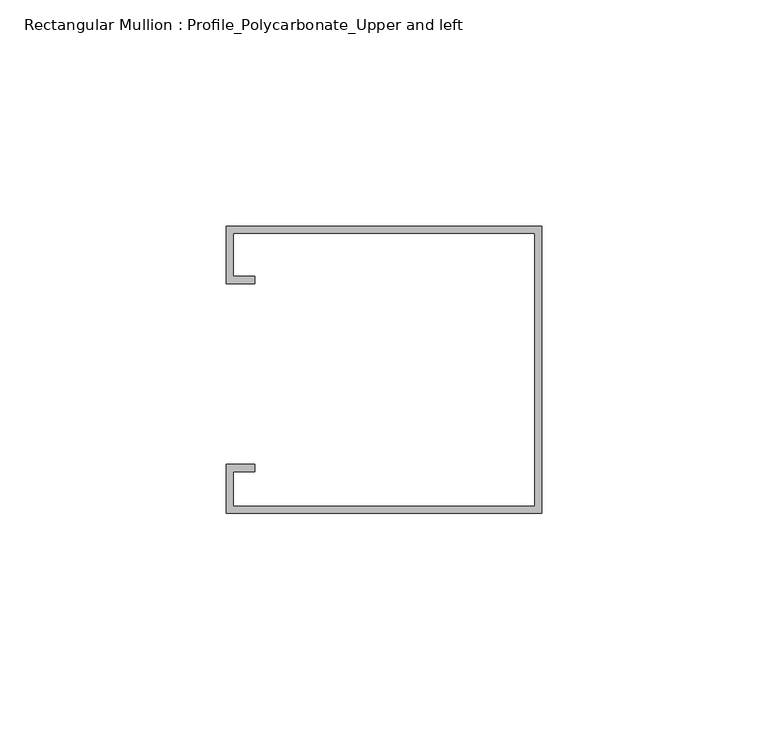
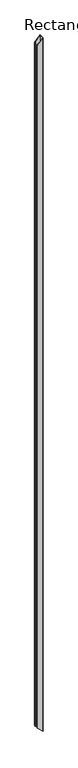
"""IFC4 building model written with IfcOpenShell, lengths in millimetres: member geometry, Rectangular Mullion : Profile_Polycarbonate_Upper and left."""

from ifc_helpers import new_model, si_unit, origin, place, context, project, spatial, faceted_brep, source, transform, mapped, element, save


def rectangular_mullion_profile_polycarbonate_upper_and_left_f935b790(model_context):
    return source(origin(), model_context, "Body", "Brep", [
        faceted_brep([(-69.85, 32.7, -75.9129484), (0.0, 32.7, 0.0), (0.0, 32.7, -9342.9603437), (-69.85, 32.7, -9278.689062), (-69.85, 20.0, -75.9129484), (-69.85, 20.0, -9278.689062), (-63.5, 20.0, -69.0117713), (-63.5, 20.0, -9284.5319058), (-63.5, 21.5875, -69.0117713), (-63.5, 21.5875, -9284.5319058), (-68.2625, 21.5875, -74.1876542), (-68.2625, 21.5875, -9280.1497729), (-68.2625, 31.1125, -74.1876542), (-68.2625, 31.1125, -9280.1497729), (-1.5875, 31.1125, -1.7252943), (-1.5875, 31.1125, -9341.4996328), (-1.5875, -29.2125, -1.7252943), (-1.5875, -29.2125, -9341.4996328), (-68.2625, -29.2125, -74.1876542), (-68.2625, -29.2125, -9280.1497729), (-68.2625, -21.5875, -74.1876542), (-68.2625, -21.5875, -9280.1497729), (-63.5, -21.5875, -69.0117713), (-63.5, -21.5875, -9284.5319058), (-63.5, -20.0, -69.0117713), (-63.5, -20.0, -9284.5319058), (-69.85, -20.0, -75.9129484), (-69.85, -20.0, -9278.689062), (-69.85, -30.8, -75.9129484), (-69.85, -30.8, -9278.689062), (0.0, -30.8, 0.0), (0.0, -30.8, -9342.9603437)], [[[0, 1, 2, 3]], [[4, 0, 3, 5]], [[6, 4, 5, 7]], [[8, 6, 7, 9]], [[10, 8, 9, 11]], [[12, 10, 11, 13]], [[14, 12, 13, 15]], [[16, 14, 15, 17]], [[18, 16, 17, 19]], [[20, 18, 19, 21]], [[22, 20, 21, 23]], [[24, 22, 23, 25]], [[26, 24, 25, 27]], [[28, 26, 27, 29]], [[30, 28, 29, 31]], [[1, 30, 31, 2]], [[1, 0, 4, 6, 8, 10, 12, 14, 16, 18, 20, 22, 24, 26, 28, 30]], [[2, 31, 29, 27, 25, 23, 21, 19, 17, 15, 13, 11, 9, 7, 5, 3]]]),
    ])


if __name__ == "__main__":
    model = new_model("IFC4")
    model_context = context("Model", 3, world=origin())
    ifc_project = project(units=[si_unit("LENGTHUNIT", "METRE", prefix="MILLI")], contexts=[model_context])
    site = spatial("IfcSite", under=ifc_project)
    building = spatial("IfcBuilding", under=site)
    placement = place(None, origin())
    rectangular_mullion_profile_polycarbonate_upper_and_left_shape = rectangular_mullion_profile_polycarbonate_upper_and_left_f935b790(model_context)
    element("IfcMember", 1, ObjectType="Rectangular Mullion : Profile_Polycarbonate_Upper and left", at=placement, inside=building, context=model_context, shape_type="MappedRepresentation", body=[
        mapped(rectangular_mullion_profile_polycarbonate_upper_and_left_shape, transform((0.0, 0.0, 0.0), x_axis=(1.0, 0.0, 0.0), y_axis=(0.0, 1.0, 0.0), z_axis=(0.0, 0.0, 1.0))),
    ])
    save(model, "model.ifc")

# Revit data of these elements
# Type "Rectangular Mullion : Profile_Polycarbonate_Upper and left"
#   built-in parameter 1007322 = 0.208333 (stored number, unit not read)
#   built-in parameter 1007321 = 0.00520833 (stored number, unit not read)
#   built-in parameter 1007320 = 0 (stored number, unit not read)
# Element 1 (IfcMember, "Rectangular Mullion : Profile_Polycarbonate_Upper and left")
#   Materials on its faces: "ALUMINUM PROFILE AT POLYCARBONATE PANEL"
# Materials
#   "ALUMINUM PROFILE AT POLYCARBONATE PANEL": class "Metal", colour RGB 244 244 244, transparency 0, Description = "Aluminum 6061", Cost = 0
